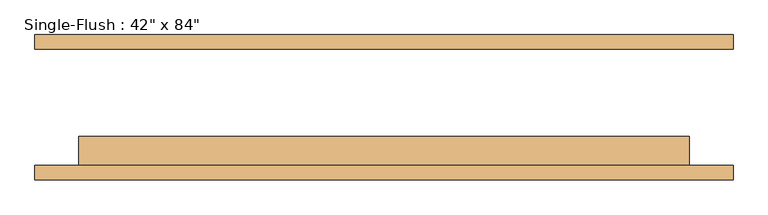
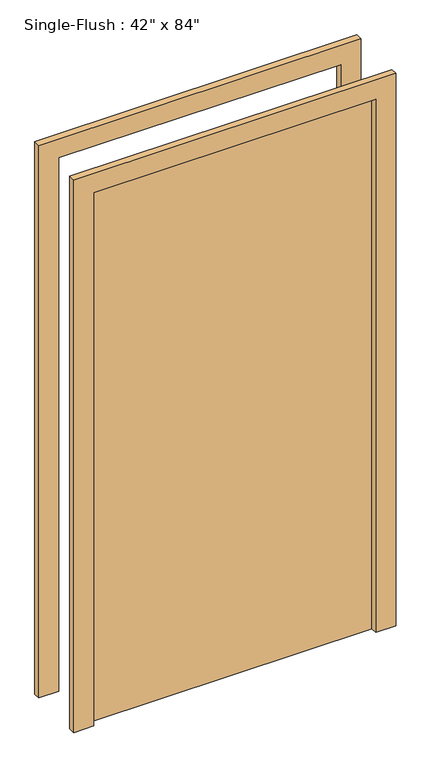
"""IFC4 building model written with IfcOpenShell, lengths in millimetres: door geometry."""

from ifc_helpers import new_model, si_unit, frame, origin, origin_with_axes, place, context, project, spatial, polyline, outline, extrude, source, transform, mapped, element, save


def door_e5858c66(model_context):
    return source(origin(), model_context, "Body", "SweptSolid", [
        extrude(outline(polyline([(2209.8, -609.6), (0.0, -609.6), (0.0, -533.4), (2133.6, -533.4), (2133.6, 533.4), (0.0, 533.4), (0.0, 609.6), (2209.8, 609.6), (2209.8, -609.6)])), frame((0.0, -127.0, 0.0), z_axis=(0.0, 1.0, 0.0), x_axis=(0.0, 0.0, 1.0)), (0.0, 0.0, 1.0), 25.4),
        extrude(outline(polyline([(2209.8, 609.6), (2209.8, -609.6), (0.0, -609.6), (0.0, -533.4), (2133.6, -533.4), (2133.6, 533.4), (0.0, 533.4), (0.0, 609.6), (2209.8, 609.6)])), frame((0.0, 101.6, 0.0), z_axis=(0.0, 1.0, 0.0), x_axis=(0.0, 0.0, 1.0)), (0.0, 0.0, 1.0), 25.4),
        extrude(outline(polyline([(533.4, -50.8), (533.4, -101.6), (-533.4, -101.6), (-533.4, -50.8), (533.4, -50.8)])), origin_with_axes(), (0.0, 0.0, 1.0), 2133.6),
    ])


if __name__ == "__main__":
    model = new_model("IFC4")
    model_context = context("Model", 3, world=origin())
    ifc_project = project(units=[si_unit("LENGTHUNIT", "METRE", prefix="MILLI")], contexts=[model_context])
    site = spatial("IfcSite", under=ifc_project)
    building = spatial("IfcBuilding", under=site)
    placement = place(None, origin())
    door_shape = door_e5858c66(model_context)
    element("IfcDoor", 1, ObjectType="Single-Flush : 42\" x 84\"", at=placement, inside=building, context=model_context, shape_type="MappedRepresentation", body=[
        mapped(door_shape, transform((0.0, 0.0, 0.0), x_axis=(1.0, 0.0, 0.0), y_axis=(0.0, 1.0, 0.0), z_axis=(0.0, 0.0, 1.0))),
    ])
    save(model, "model.ifc")

# Revit data of these elements
# Type "Single-Flush : 42\" x 84\""
#   Type Mark = "9"
#   Construction Type = "B"
#   Assembly Code = "C1020"
#   Thickness = 0' - 2"
#   Height = 7' - 0"
#   Trim Projection Ext = 0' - 1"
#   Trim Projection Int = 0' - 1"
#   Trim Width = 0' - 3"
#   Width = 3' - 6"
#   Door Material = Door - Panel
#   Frame Material = Door - Frame
#   Function = (empty or 0)
#   Wall Closure = (empty or 0)
# Element 1 (IfcDoor, "Single-Flush : 42\" x 84\"")
#   Materials on its faces: "Door - Frame", "Door - Panel"
# Materials
#   "Door - Panel": class "Wood", colour RGB 210 159 95, transparency 0
#   "Door - Frame": class "Miscellaneous", colour RGB 118 70 51, transparency 0
